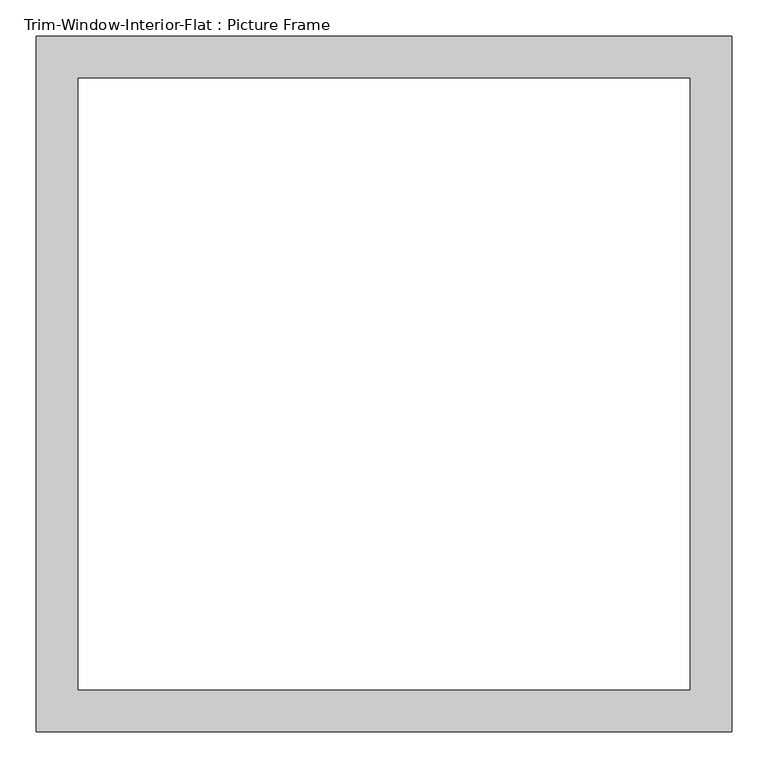
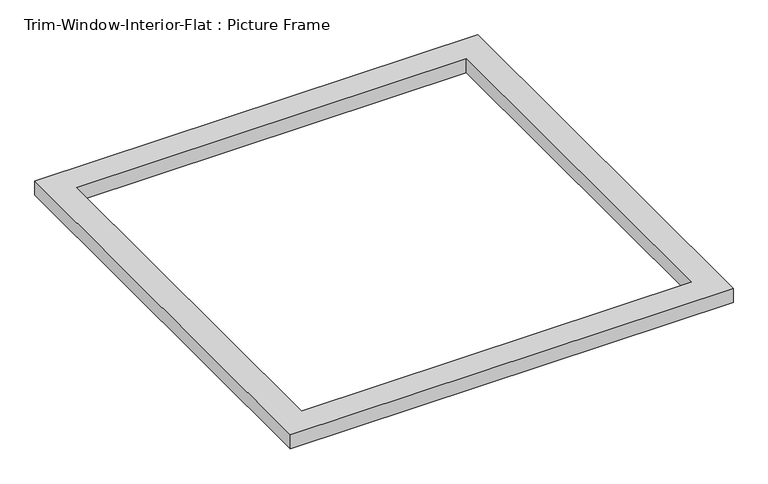
"""IFC4 building model written with IfcOpenShell, lengths in millimetres: proxy geometry, Trim-Window-Interior-Flat : Picture Frame."""

import ifcopenshell
import ifcopenshell.guid

model = None  # the IFC model being written
_history = None  # IfcOwnerHistory: only IFC2X3 demands one
_inside = {}  # id of a spatial element -> (the spatial element, [elements in it])
_under = {}  # id of a project, library or spatial element -> (it, [spatial elements below it])
_declared = {}  # id of a project -> (the project, [libraries it declares])
_typed = {}  # id of a type object -> (the type object, [elements of that type])
_made_of = {}  # id of a material, layer set ... -> (it, [elements and type objects made of it])


def new_model(schema):
    """Start an empty IFC model of exactly this schema.

    Asked for "IFC4X3", IfcOpenShell would pick the latest addendum, in which some entities
    have other attributes; the version numbers below select the first issue.
    IFC2X3 requires an IfcOwnerHistory on every rooted entity: one is made here for all.
    """
    global model, _history
    if schema == "IFC4X3":
        model = ifcopenshell.file(schema_version=(4, 3, 0, 0))
    else:
        model = ifcopenshell.file(schema=schema)
    _inside.clear()
    _under.clear()
    _declared.clear()
    _typed.clear()
    _made_of.clear()
    _history = None
    if model.schema == "IFC2X3":
        org = make("IfcOrganization", Name="unknown")
        user = make(
            "IfcPersonAndOrganization",
            ThePerson=make("IfcPerson", FamilyName="unknown"),
            TheOrganization=org,
        )
        app = make(
            "IfcApplication",
            ApplicationDeveloper=org,
            Version="unknown",
            ApplicationFullName="unknown",
            ApplicationIdentifier="unknown",
        )
        _history = make(
            "IfcOwnerHistory",
            OwningUser=user,
            OwningApplication=app,
            ChangeAction="ADDED",
            CreationDate=0,
        )
    return model


def make(cls, **values):
    """One entity of the class cls with the attributes given. An attribute that is None is left unset."""
    return model.create_entity(
        cls, **{name: value for name, value in values.items() if value is not None}
    )


def rooted(cls, **values):
    """An entity with a GlobalId (a new one), such as an element, a storey or a relation."""
    return make(cls, GlobalId=ifcopenshell.guid.new(), OwnerHistory=_history, **values)


def si_unit(unit_type, name, prefix=None):
    """IfcSIUnit, for example si_unit("LENGTHUNIT", "METRE", prefix="MILLI")."""
    return make("IfcSIUnit", UnitType=unit_type, Prefix=prefix, Name=name)


def assignment(units):
    """IfcUnitAssignment: the units of a project."""
    return None if units is None else make("IfcUnitAssignment", Units=units)


def point(xyz):
    """IfcCartesianPoint."""
    return None if xyz is None else make("IfcCartesianPoint", Coordinates=xyz)


def direction(xyz):
    """IfcDirection."""
    return None if xyz is None else make("IfcDirection", DirectionRatios=xyz)


def frame(location, z_axis=None, x_axis=None):
    """IfcAxis2Placement3D, a coordinate frame: its origin and axes. An axis left out is left unset."""
    return make(
        "IfcAxis2Placement3D",
        Location=point(location),
        Axis=direction(z_axis),
        RefDirection=direction(x_axis),
    )


def origin():
    """The frame at (0, 0, 0) with its axes left unset."""
    return frame((0.0, 0.0, 0.0))


def origin_with_axes():
    """The frame at (0, 0, 0) with the z axis (0, 0, 1) and the x axis (1, 0, 0) written out."""
    return frame((0.0, 0.0, 0.0), z_axis=(0.0, 0.0, 1.0), x_axis=(1.0, 0.0, 0.0))


def place(relative_to, where):
    """IfcLocalPlacement: puts the frame where relative to a parent placement (None: the world)."""
    return make(
        "IfcLocalPlacement", PlacementRelTo=relative_to, RelativePlacement=where
    )


def context(
    kind, dimensions, precision=None, world=None, true_north=None, identifier=None
):
    """IfcGeometricRepresentationContext, for example the 3D "Model" context."""
    return make(
        "IfcGeometricRepresentationContext",
        ContextIdentifier=identifier,
        ContextType=kind,
        CoordinateSpaceDimension=dimensions,
        Precision=precision,
        WorldCoordinateSystem=world,
        TrueNorth=true_north,
    )


def project(units=None, contexts=None):
    """IfcProject with its units and contexts."""
    return rooted(
        "IfcProject",
        Name="project",
        RepresentationContexts=contexts,
        UnitsInContext=assignment(units),
    )


def spatial(cls, under=None, at=None, **own):
    """A site, building, storey or space (cls), placed at a placement, below another one or the project."""
    s = rooted(cls, ObjectPlacement=at, **own)
    if under is not None:
        _under.setdefault(under.id(), (under, []))[1].append(s)
    return s


def polyline(points):
    """IfcPolyline through the points."""
    return make("IfcPolyline", Points=[point(p) for p in points])


def outline(outer, holes=None, kind="AREA"):
    """IfcArbitraryClosedProfileDef: a profile drawn as a closed curve; with holes, ...WithVoids."""
    if holes is None:
        return make("IfcArbitraryClosedProfileDef", ProfileType=kind, OuterCurve=outer)
    return make(
        "IfcArbitraryProfileDefWithVoids",
        ProfileType=kind,
        OuterCurve=outer,
        InnerCurves=holes,
    )


def extrude(swept, where, along, depth):
    """IfcExtrudedAreaSolid: the profile swept, set in the frame where, extruded along a direction by depth."""
    return make(
        "IfcExtrudedAreaSolid",
        SweptArea=swept,
        Position=where,
        ExtrudedDirection=direction(along),
        Depth=depth,
    )


def shape(context_of_items, identifier, shape_type, items):
    """IfcShapeRepresentation: the items that make up one representation, for example the "Body"."""
    return make(
        "IfcShapeRepresentation",
        ContextOfItems=context_of_items,
        RepresentationIdentifier=identifier,
        RepresentationType=shape_type,
        Items=items,
    )


def source(mapping_origin, context_of_items, identifier, shape_type, items):
    """IfcRepresentationMap: a shape defined once, which mapped items show again and again."""
    return make(
        "IfcRepresentationMap",
        MappingOrigin=mapping_origin,
        MappedRepresentation=shape(context_of_items, identifier, shape_type, items),
    )


def transform(
    local_origin,
    x_axis=None,
    y_axis=None,
    z_axis=None,
    scale=None,
    scale2=None,
    scale3=None,
    uniform=True,
):
    """IfcCartesianTransformationOperator3D, or its non-uniform kind. x_axis, y_axis, z_axis: its Axis1, 2, 3."""
    if uniform:
        return make(
            "IfcCartesianTransformationOperator3D",
            Axis1=direction(x_axis),
            Axis2=direction(y_axis),
            LocalOrigin=point(local_origin),
            Scale=scale,
            Axis3=direction(z_axis),
        )
    return make(
        "IfcCartesianTransformationOperator3DnonUniform",
        Axis1=direction(x_axis),
        Axis2=direction(y_axis),
        LocalOrigin=point(local_origin),
        Scale=scale,
        Axis3=direction(z_axis),
        Scale2=scale2,
        Scale3=scale3,
    )


def mapped(mapping_source, mapping_target):
    """IfcMappedItem: shows the shape of a source again, moved by a transform."""
    return make(
        "IfcMappedItem", MappingSource=mapping_source, MappingTarget=mapping_target
    )


def made_of(thing, what):
    """Note that an element or type object is made of a material, layer set ...; save() writes the relation."""
    if what is not None:
        _made_of.setdefault(what.id(), (what, []))[1].append(thing)
    return thing


def element(
    cls,
    number,
    at=None,
    inside=None,
    cuts=None,
    type_object=None,
    material=None,
    context=None,
    identifier="Body",
    shape_type=None,
    held_by="IfcProductDefinitionShape",
    body=None,
    shapes=None,
    **own,
):
    """One element of the class cls, such as IfcWall. Its Tag is "e" and its number.

    at: its placement. inside: the storey or other place that contains it. cuts: it is an
    opening in that element (IfcRelVoidsElement). A single representation is given by context,
    identifier, shape_type and body (its items); several are given by shapes. held_by: the class
    of the entity that holds the representations. save() writes the other relations.
    """
    e = rooted(cls, Tag="e%d" % number, ObjectPlacement=at, **own)
    if body is not None:
        shapes = [shape(context, identifier, shape_type, body)]
    if shapes is not None:
        e.Representation = make(held_by, Representations=shapes)
    if inside is not None:
        _inside.setdefault(inside.id(), (inside, []))[1].append(e)
    if cuts is not None:
        rooted(
            "IfcRelVoidsElement", RelatingBuildingElement=cuts, RelatedOpeningElement=e
        )
    if type_object is not None:
        _typed.setdefault(type_object.id(), (type_object, []))[1].append(e)
    return made_of(e, material)


def aggregate(whole, parts):
    """IfcRelAggregates: a whole, such as a stair, and the parts it consists of."""
    return rooted("IfcRelAggregates", RelatingObject=whole, RelatedObjects=parts)


def save(model, path):
    """Write the relations noted so far, then the file.

    IfcRelAggregates (storeys below a building ...), IfcRelContainedInSpatialStructure (elements
    in a storey), IfcRelDefinesByType, IfcRelAssociatesMaterial and IfcRelDeclares: one each for
    every whole, place, type object, material and project.
    """
    for whole, parts in _under.values():
        aggregate(whole, parts)
    for where, things in _inside.values():
        rooted(
            "IfcRelContainedInSpatialStructure",
            RelatedElements=things,
            RelatingStructure=where,
        )
    for kind, things in _typed.values():
        rooted("IfcRelDefinesByType", RelatedObjects=things, RelatingType=kind)
    for what, things in _made_of.values():
        rooted("IfcRelAssociatesMaterial", RelatedObjects=things, RelatingMaterial=what)
    for by, libraries in _declared.values():
        rooted("IfcRelDeclares", RelatingContext=by, RelatedDefinitions=libraries)
    model.write(path)


def trim_window_interior_flat_picture_frame_8ff237ef(model_context):
    return source(origin(), model_context, "Body", "SweptSolid", [
        extrude(outline(polyline([(476.25, 44.45), (476.25, -908.05), (-476.25, -908.05), (-476.25, 44.45), (476.25, 44.45)]), holes=[polyline([(419.1, -12.7), (-419.1, -12.7), (-419.1, -850.9), (419.1, -850.9), (419.1, -12.7)])]), origin_with_axes(), (0.0, 0.0, 1.0), 31.75),
    ])


if __name__ == "__main__":
    model = new_model("IFC4")
    model_context = context("Model", 3, world=origin())
    ifc_project = project(units=[si_unit("LENGTHUNIT", "METRE", prefix="MILLI")], contexts=[model_context])
    site = spatial("IfcSite", under=ifc_project)
    building = spatial("IfcBuilding", under=site)
    placement = place(None, origin())
    trim_window_interior_flat_picture_frame_shape = trim_window_interior_flat_picture_frame_8ff237ef(model_context)
    element("IfcBuildingElementProxy", 1, Name="Trim-Window-Interior-Flat : Picture Frame", ObjectType="Trim-Window-Interior-Flat : Picture Frame", at=placement, inside=building, context=model_context, shape_type="MappedRepresentation", body=[
        mapped(trim_window_interior_flat_picture_frame_shape, transform((0.0, 0.0, 0.0), x_axis=(1.0, 0.0, 0.0), y_axis=(0.0, 1.0, 0.0), z_axis=(0.0, 0.0, 1.0))),
    ])
    save(model, "model.ifc")

# Revit data of these elements
# Type "Trim-Window-Interior-Flat : Picture Frame"
#   Trim Thickness_Picture Frame = 0' - 1 1/4"
#   Trim Width = 0' - 2 1/4"
#   Trim Thickness_with Sill = 0' - 0 3/4"
#   Sill Thickness = 0' - 1 1/4"
#   Opening Width [instance default] = 2' - 0"
#   Opening Height [instance default] = 3' - 0"
#   Default Elevation = 4' - 0"
#   Sill = no
#   Picture Frame = yes
#   Trim Material [instance default] = none
# Element 1 (IfcBuildingElementProxy, "Trim-Window-Interior-Flat : Picture Frame")
#   Opening Width = 2' - 10"
#   Opening Height = 2' - 10"
#   Trim Material = Wood - Stained
#   Materials on its faces: "Wood - Stained"
# Materials
#   "Wood - Stained": class "Wood", colour RGB 224 178 126, transparency 0, Cost = 0
